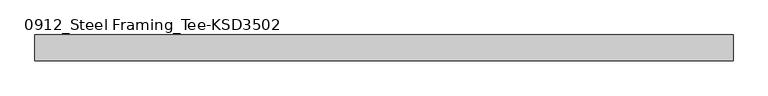
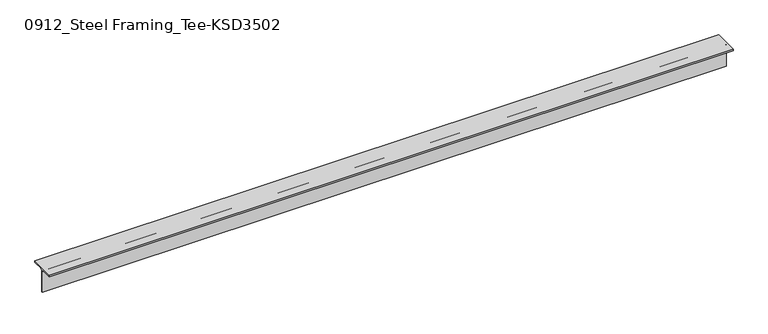
"""IFC4 building model written with IfcOpenShell, lengths in millimetres: member geometry, 0912_Steel Framing_Tee-KSD3502 : H_SB_ASB_CT-150x150x6.5x9."""

from ifc_helpers import new_model, si_unit, point, frame, frame_2d, origin, place, context, project, spatial, polyline, circle_curve, trimmed, segment, composite_curve, outline, extrude, source, transform, mapped, element, save


def member_0912_steel_framing_tee_ksd3502_76157bc4(model_context):
    return source(origin(), model_context, "Body", "SweptSolid", [
        extrude(outline(composite_curve([segment(polyline([(-75.0, 75.0), (75.0, 75.0), (75.0, 66.0), (16.25, 66.0)]), True, "CONTINUOUS"), segment(trimmed(circle_curve(frame_2d((16.25, 53.0)), 13.0), [point((16.25, 66.0))], [point((3.25, 53.0))], True, "CARTESIAN"), True, "CONTINUOUS"), segment(polyline([(3.25, 53.0), (3.25, -75.0), (-3.25, -75.0), (-3.25, 53.0)]), True, "CONTINUOUS"), segment(trimmed(circle_curve(frame_2d((-16.25, 53.0)), 13.0), [point((-3.25, 53.0))], [point((-16.25, 66.0))], True, "CARTESIAN"), True, "CONTINUOUS"), segment(polyline([(-16.25, 66.0), (-75.0, 66.0), (-75.0, 75.0)]), True, "CONTINUOUS")], self_intersect=False)), frame((-2028.8, 0.0, 0.0), z_axis=(1.0, 0.0, 0.0), x_axis=(0.0, 1.0, 0.0)), (0.0, 0.0, 1.0), 4074.9),
    ])


if __name__ == "__main__":
    model = new_model("IFC4")
    model_context = context("Model", 3, world=origin())
    ifc_project = project(units=[si_unit("LENGTHUNIT", "METRE", prefix="MILLI")], contexts=[model_context])
    site = spatial("IfcSite", under=ifc_project)
    building = spatial("IfcBuilding", under=site)
    placement = place(None, origin())
    member_0912_steel_framing_tee_ksd3502_shape = member_0912_steel_framing_tee_ksd3502_76157bc4(model_context)
    element("IfcMember", 1, ObjectType="0912_Steel Framing_Tee-KSD3502 : H_SB_ASB_CT-150x150x6.5x9", at=placement, inside=building, context=model_context, shape_type="MappedRepresentation", body=[
        mapped(member_0912_steel_framing_tee_ksd3502_shape, transform((0.0, 0.0, 0.0), x_axis=(1.0, 0.0, 0.0), y_axis=(0.0, 1.0, 0.0), z_axis=(0.0, 0.0, 1.0))),
    ])
    save(model, "model.ifc")

# Revit data of these elements
# Type "0912_Steel Framing_Tee-KSD3502 : H_SB_ASB_CT-150x150x6.5x9"
#   H_WM Code_1 = "S01AA003-00001 | Main Steel Structure Fabrication Work | Shelter/Building | Light Steel - Standard (30KG/M>Weight) | Material: (   )"
#   H_WM Code_2 = "S03AA029-00001 | Main Steel Structure Erection Work | Shelter/Building | Light Steel (30KG/M>Weight) | Material: (   )"
#   H_WM Code_3 = "S01AA010-00001 | Main Steel Structure Fabrication Work | Shelter/Building | Steel Painting/Coating | for Non-Fireproofed Steel Surface, Surface Preparation, Primer, Second & Final Coat | Material: (   )"
#   H_Q'ty Cal Type Tag = "SB-Q2"
#   Width = 15.0 cm
#   Web Thickness = 0.65 cm
#   Web Fillet = 1.3 cm
#   Section Area = 23.39 cm²
#   Perimeter = 0.60 m²/m
#   Nominal Weight = 18.40 kgf/m
#   Height = 15.0 cm
#   Flange Thickness = 0.9 cm
#   Centroid Vertical = 7.5 cm
#   Centroid Horizontal = 7.5 cm
#   Length [instance default] = 1.5000 m
#   Structural Material [instance default] = Steel, 45-345
#   Warping Constant = (empty or 0)
#   Torsional Moment of Inertia = 0
#   Section Name Key = ""
#   Plastic Modulus weak axis = 0
#   Plastic Modulus strong axis = 0
#   Moment of Inertia weak axis = 0
#   Moment of Inertia strong axis = 0
#   Elastic Modulus weak axis = 0
#   Elastic Modulus strong axis = 0
#   Bolt Spacing = 0
#   Assembly Code = ""
# Element 1 (IfcMember, "0912_Steel Framing_Tee-KSD3502 : H_SB_ASB_CT-150x150x6.5x9")
#   Structural Material = none
# Materials
#   "Steel, 45-345": class "Metal", colour RGB 189 187 185, transparency 0, Description = "Steel 345 MPa", Cost = 0
